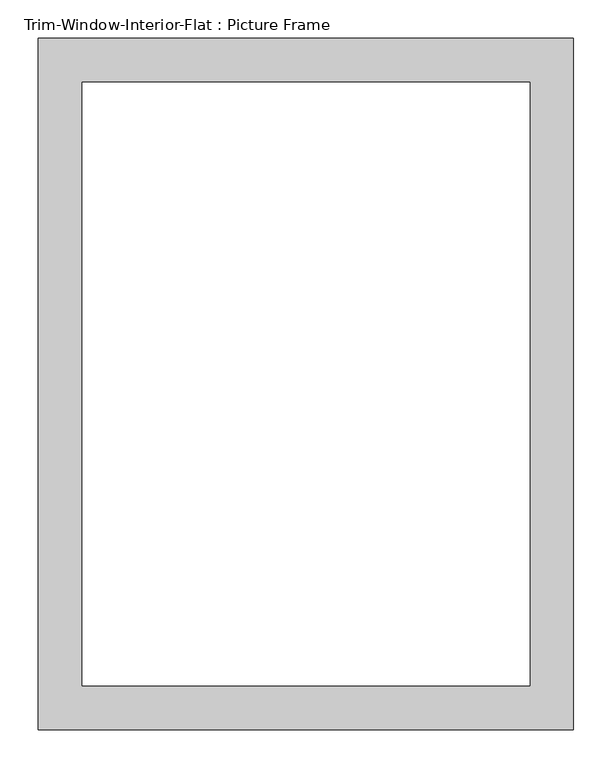
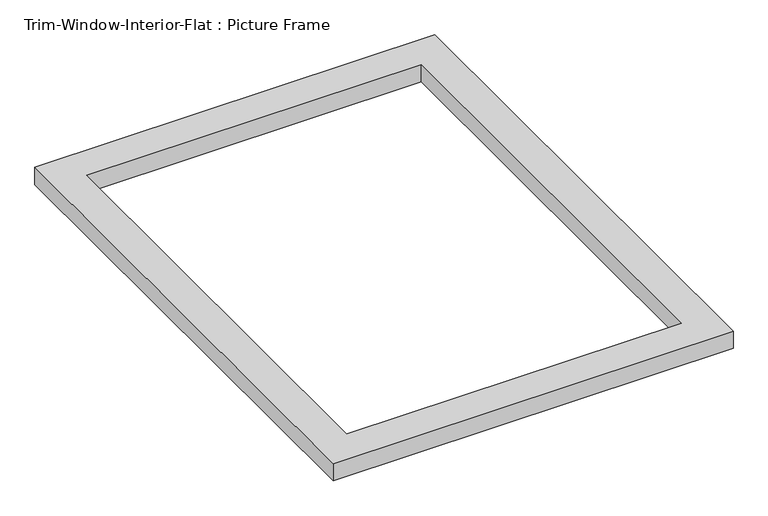
"""IFC4 building model written with IfcOpenShell, lengths in millimetres: proxy geometry, Trim-Window-Interior-Flat : Picture Frame."""

from ifc_helpers import new_model, si_unit, origin, origin_with_axes, place, context, project, spatial, polyline, outline, extrude, source, transform, mapped, element, save


def trim_window_interior_flat_picture_frame_6a74a1f9(model_context):
    return source(origin(), model_context, "Body", "SweptSolid", [
        extrude(outline(polyline([(349.25, 44.45), (349.25, -857.25), (-349.25, -857.25), (-349.25, 44.45), (349.25, 44.45)]), holes=[polyline([(292.1, -12.7), (-292.1, -12.7), (-292.1, -800.1), (292.1, -800.1), (292.1, -12.7)])]), origin_with_axes(), (0.0, 0.0, 1.0), 31.75),
    ])


if __name__ == "__main__":
    model = new_model("IFC4")
    model_context = context("Model", 3, world=origin())
    ifc_project = project(units=[si_unit("LENGTHUNIT", "METRE", prefix="MILLI")], contexts=[model_context])
    site = spatial("IfcSite", under=ifc_project)
    building = spatial("IfcBuilding", under=site)
    placement = place(None, origin())
    trim_window_interior_flat_picture_frame_shape = trim_window_interior_flat_picture_frame_6a74a1f9(model_context)
    element("IfcBuildingElementProxy", 1, Name="Trim-Window-Interior-Flat : Picture Frame", ObjectType="Trim-Window-Interior-Flat : Picture Frame", at=placement, inside=building, context=model_context, shape_type="MappedRepresentation", body=[
        mapped(trim_window_interior_flat_picture_frame_shape, transform((0.0, 0.0, 0.0), x_axis=(1.0, 0.0, 0.0), y_axis=(0.0, 1.0, 0.0), z_axis=(0.0, 0.0, 1.0))),
    ])
    save(model, "model.ifc")

# Revit data of these elements
# Type "Trim-Window-Interior-Flat : Picture Frame"
#   Trim Thickness_Picture Frame = 0' - 1 1/4"
#   Trim Width = 0' - 2 1/4"
#   Trim Thickness_with Sill = 0' - 0 3/4"
#   Sill Thickness = 0' - 1 1/4"
#   Opening Width [instance default] = 2' - 0"
#   Opening Height [instance default] = 3' - 0"
#   Default Elevation = 4' - 0"
#   Sill = no
#   Picture Frame = yes
#   Trim Material [instance default] = none
# Element 1 (IfcBuildingElementProxy, "Trim-Window-Interior-Flat : Picture Frame")
#   Opening Height = 2' - 8"
#   Trim Material = Wood - Stained
#   Materials on its faces: "Wood - Stained"
# Materials
#   "Wood - Stained": class "Wood", colour RGB 224 178 126, transparency 0, Cost = 0
